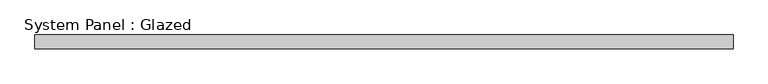
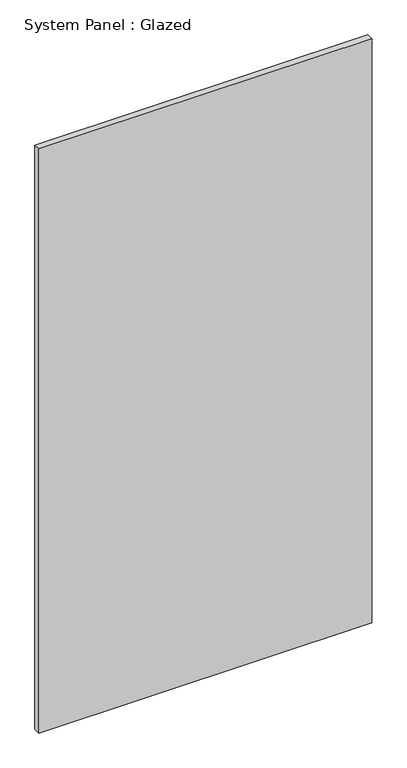
"""IFC4 building model written with IfcOpenShell, lengths in millimetres: plate geometry, System Panel : Glazed."""

from ifc_helpers import new_model, si_unit, origin, origin_with_axes, place, context, project, spatial, polyline, outline, extrude, source, transform, mapped, element, save


def system_panel_glazed_b60b372a(model_context):
    return source(origin(), model_context, "Body", "SweptSolid", [
        extrude(outline(polyline([(626.7857144, 24.5), (-626.7857144, 24.5), (-626.7857144, 49.5), (626.7857144, 49.5), (626.7857144, 24.5)])), origin_with_axes(), (0.0, 0.0, 1.0), 2325.0),
    ])


if __name__ == "__main__":
    model = new_model("IFC4")
    model_context = context("Model", 3, world=origin())
    ifc_project = project(units=[si_unit("LENGTHUNIT", "METRE", prefix="MILLI")], contexts=[model_context])
    site = spatial("IfcSite", under=ifc_project)
    building = spatial("IfcBuilding", under=site)
    placement = place(None, origin())
    system_panel_glazed_shape = system_panel_glazed_b60b372a(model_context)
    element("IfcPlate", 1, ObjectType="System Panel : Glazed", at=placement, inside=building, context=model_context, shape_type="MappedRepresentation", body=[
        mapped(system_panel_glazed_shape, transform((0.0, 0.0, 0.0), x_axis=(1.0, 0.0, 0.0), y_axis=(0.0, 1.0, 0.0), z_axis=(0.0, 0.0, 1.0))),
    ])
    save(model, "model.ifc")

# Revit data of these elements
# Type "System Panel : Glazed"
#   Construction Type Id = "GSP4R"
#   Analytic Construction = "1/8 in Pilkington single glazing"
#   Visual Light Transmittance = 0.9
#   Solar Heat Gain Coefficient = 0.86
#   Heat Transfer Coefficient (U) = 6.7069 W/(m²·K)
#   Define Thermal Properties by = 1
# Element 1 (IfcPlate, "System Panel : Glazed")
#   Materials on its faces: "Glass"
# Materials
#   "Glass": class "Glass", colour RGB 0 128 192, transparency 0.75, Description = "Soda Lime Glass", Cost = 0
